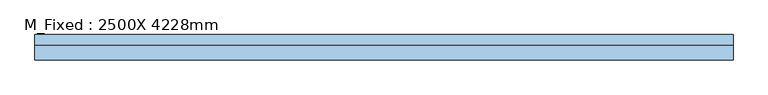
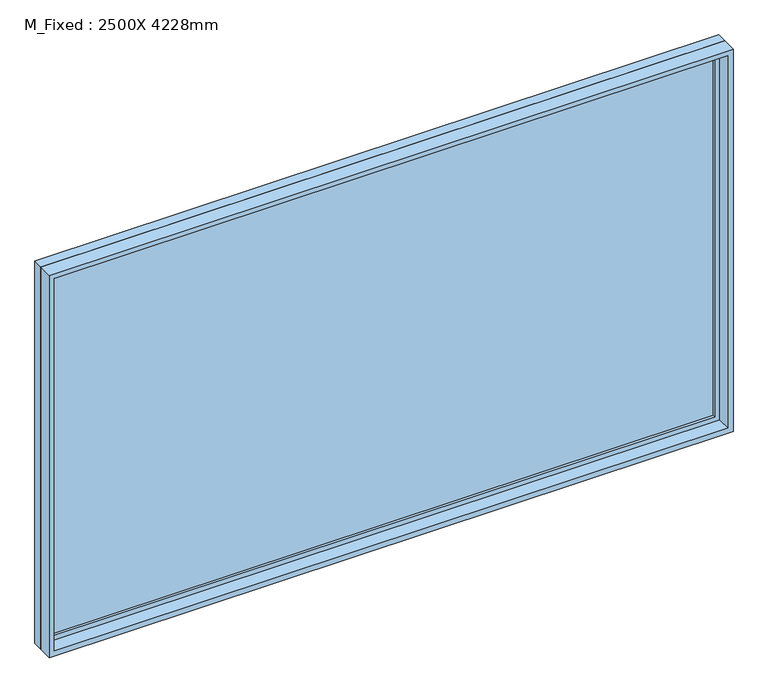
"""IFC4 building model written with IfcOpenShell, lengths in millimetres: window geometry, M_Fixed : 2500X 4228mm."""

from ifc_helpers import new_model, si_unit, frame, origin, place, context, project, spatial, polyline, outline, extrude, source, transform, mapped, element, save


def m_fixed_2500x_4228mm_fd5e51e7(model_context):
    return source(origin(), model_context, "Body", "SweptSolid", [
        extrude(outline(polyline([(-2050.8, 54.2), (2050.8, 54.2), (2050.8, 42.2), (-2050.8, 42.2), (-2050.8, 54.2)])), frame((0.0, 0.0, 368.0), z_axis=(0.0, 0.0, 1.0), x_axis=(1.0, 0.0, 0.0)), (0.0, 0.0, 1.0), 2374.0),
        extrude(outline(polyline([(2786.0, -2094.8), (324.0, -2094.8), (324.0, 2094.8), (2786.0, 2094.8), (2786.0, -2094.8)]), holes=[polyline([(2742.0, -2050.8), (2742.0, 2050.8), (368.0, 2050.8), (368.0, -2050.8), (2742.0, -2050.8)])]), frame((0.0, 26.2, 0.0), z_axis=(0.0, 1.0, 0.0), x_axis=(0.0, 0.0, 1.0)), (0.0, 0.0, 1.0), 44.0),
        extrude(outline(polyline([(2805.0, -2113.8), (305.0, -2113.8), (305.0, 2113.8), (2805.0, 2113.8), (2805.0, -2113.8)]), holes=[polyline([(2786.0, -2094.8), (2786.0, 2094.8), (324.0, 2094.8), (324.0, -2094.8), (2786.0, -2094.8)])]), frame((0.0, 26.2, 0.0), z_axis=(0.0, 1.0, 0.0), x_axis=(0.0, 0.0, 1.0)), (0.0, 0.0, 1.0), 63.0),
        extrude(outline(polyline([(2805.0, -2113.8), (305.0, -2113.8), (305.0, 2113.8), (2805.0, 2113.8), (2805.0, -2113.8)]), holes=[polyline([(2773.0, -2081.8), (2773.0, 2081.8), (337.0, 2081.8), (337.0, -2081.8), (2773.0, -2081.8)])]), frame((0.0, -63.2, 0.0), z_axis=(0.0, 1.0, 0.0), x_axis=(0.0, 0.0, 1.0)), (0.0, 0.0, 1.0), 89.4),
    ])


if __name__ == "__main__":
    model = new_model("IFC4")
    model_context = context("Model", 3, world=origin())
    ifc_project = project(units=[si_unit("LENGTHUNIT", "METRE", prefix="MILLI")], contexts=[model_context])
    site = spatial("IfcSite", under=ifc_project)
    building = spatial("IfcBuilding", under=site)
    placement = place(None, origin())
    m_fixed_2500x_4228mm_shape = m_fixed_2500x_4228mm_fd5e51e7(model_context)
    element("IfcWindow", 1, ObjectType="M_Fixed : 2500X 4228mm", at=placement, inside=building, context=model_context, shape_type="MappedRepresentation", body=[
        mapped(m_fixed_2500x_4228mm_shape, transform((0.0, 0.0, 0.0), x_axis=(1.0, 0.0, 0.0), y_axis=(0.0, 1.0, 0.0), z_axis=(0.0, 0.0, 1.0))),
    ])
    save(model, "model.ifc")

# Revit data of these elements
# Type "M_Fixed : 2500X 4228mm"
#   Type Mark = "25"
#   Height = 2500 mm
#   Default Sill Height = 305 mm
#   Width = 4227.6 mm
#   Window Inset = 19 mm
#   Frame Exterior Material = Sash
#   Frame Interior Material = Sash
#   Glass Pane Material = Glass
#   Sash = Sash
#   Wall Closure = (empty or 0)
# Element 1 (IfcWindow, "M_Fixed : 2500X 4228mm")
#   Materials on its faces: "Sash", "Glass"
# Materials
#   "Sash": class "Wood", colour RGB 136 99 55, transparency 0
#   "Glass": class "Glass", colour RGB 0 128 192, transparency 0.9, Description = "Soda Lime Glass", Cost = 0
